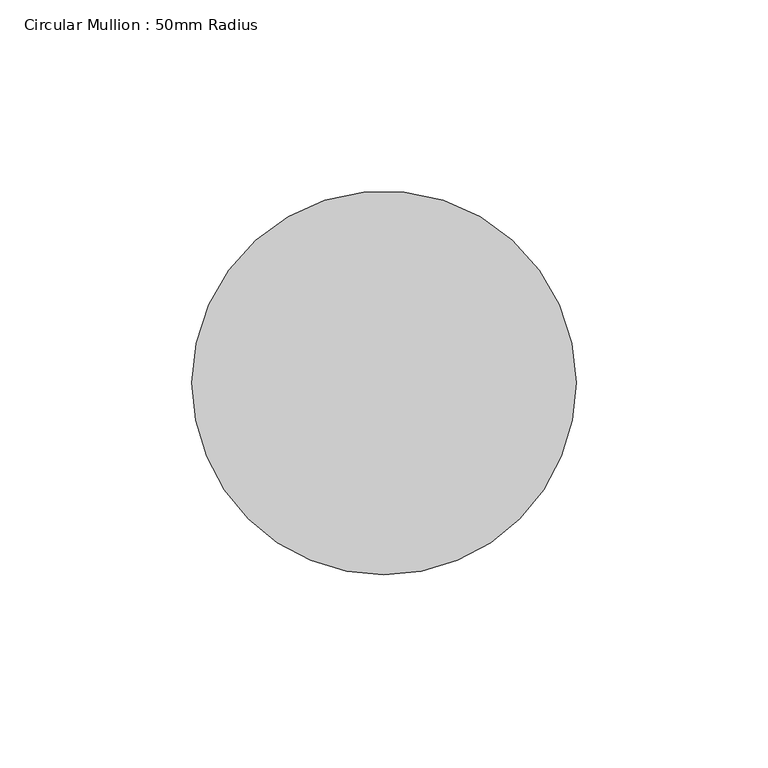
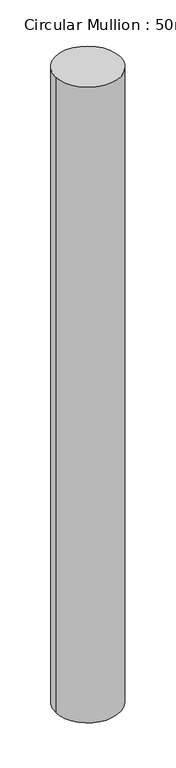
"""IFC4 building model written with IfcOpenShell, lengths in millimetres: member geometry, Circular Mullion : 50mm Radius."""

from ifc_helpers import new_model, si_unit, frame, origin, place, context, project, spatial, ellipse_curve, source, transform, mapped, element, save
from ifc_brep_helpers import plane_surface, cylinder_surface, advanced_brep


def circular_mullion_50mm_radius_fe3b235b(model_context):
    return source(origin(), model_context, "Body", "AdvancedBrep", [
        advanced_brep(
        [(-100.0, 0.0, 1.4061039), (0.0, 0.0, 0.0), (0.0, 0.0, -1040.2388389), (-100.0, 0.0, -1041.6076484)],
        [
            (0, 1, ellipse_curve(frame((-50.0, 0.0, 0.703052), z_axis=(-0.014058083331728985, -0.014924385542299667, -0.9997897944114168), x_axis=(-0.6855205996420267, -0.7277644814606294, 0.02050285323502297)), 50.0105125, 50.0)),
            (1, 2),
            (2, 3, ellipse_curve(frame((-50.0, 0.0, -1040.9232437), z_axis=(-0.01368536833914133, -0.014528702708762954, 0.999800793903977), x_axis=(0.6855281416061615, 0.727772488183653, 0.019959271253652298)), 50.0099623, 50.0)),
            (3, 0),
            (1, 0, ellipse_curve(frame((-50.0, 0.0, 0.703052), z_axis=(-0.014058083331728985, -0.014924385542299667, -0.9997897944114168), x_axis=(-0.6855205996420267, -0.7277644814606294, 0.02050285323502297)), 50.0105125, 50.0)),
            (3, 2, ellipse_curve(frame((-50.0, 0.0, -1040.9232437), z_axis=(-0.01368536833914133, -0.014528702708762954, 0.999800793903977), x_axis=(0.6855281416061615, 0.727772488183653, 0.019959271253652298)), 50.0099623, 50.0)),
        ],
        [
            cylinder_surface(frame((-50.0, 0.0, 0.0), z_axis=(0.0, 0.0, 1.0), x_axis=(1.0, 0.0, 0.0)), 50.0),
            plane_surface(frame((-221.8692521, 208.9906098, 0.0), z_axis=(0.014058083331728989, 0.01492438554229967, 0.999789794411417), x_axis=(0.6855205996420278, 0.7277644814606287, -0.020502853235026576))),
            plane_surface(frame((-221.8692521, 208.9906098, -1040.2388389), z_axis=(0.013685368339141326, 0.01452870270876295, -0.9998007939039768), x_axis=(0.6855281416061614, 0.7277724881836529, 0.019959271253670252))),
        ],
        [
            (0, [[1, 2, 3, 4]]),
            (0, [[5, -4, 6, -2]]),
            (1, [[-1, -5]]),
            (2, [[-6, -3]]),
        ],
    ),
    ])


if __name__ == "__main__":
    model = new_model("IFC4")
    model_context = context("Model", 3, world=origin())
    ifc_project = project(units=[si_unit("LENGTHUNIT", "METRE", prefix="MILLI")], contexts=[model_context])
    site = spatial("IfcSite", under=ifc_project)
    building = spatial("IfcBuilding", under=site)
    placement = place(None, origin())
    circular_mullion_50mm_radius_shape = circular_mullion_50mm_radius_fe3b235b(model_context)
    element("IfcMember", 1, ObjectType="Circular Mullion : 50mm Radius", at=placement, inside=building, context=model_context, shape_type="MappedRepresentation", body=[
        mapped(circular_mullion_50mm_radius_shape, transform((0.0, 0.0, 0.0), x_axis=(1.0, 0.0, 0.0), y_axis=(0.0, 1.0, 0.0), z_axis=(0.0, 0.0, 1.0))),
    ])
    save(model, "model.ifc")

# Revit data of these elements
# Type "Circular Mullion : 50mm Radius"
#   built-in parameter 1007350 = 0.164042 (stored number, unit not read)
# Element 1 (IfcMember, "Circular Mullion : 50mm Radius")
#   Materials on its faces: "Aluminium"
# Materials
#   "Aluminium": class "Metal", colour RGB 247 247 247, transparency 0, Description = "Aluminium 6061", Cost = 0
